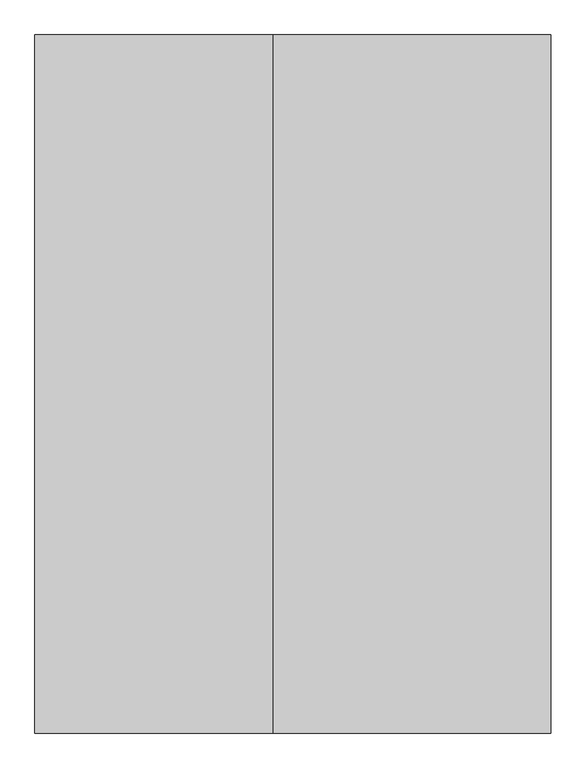
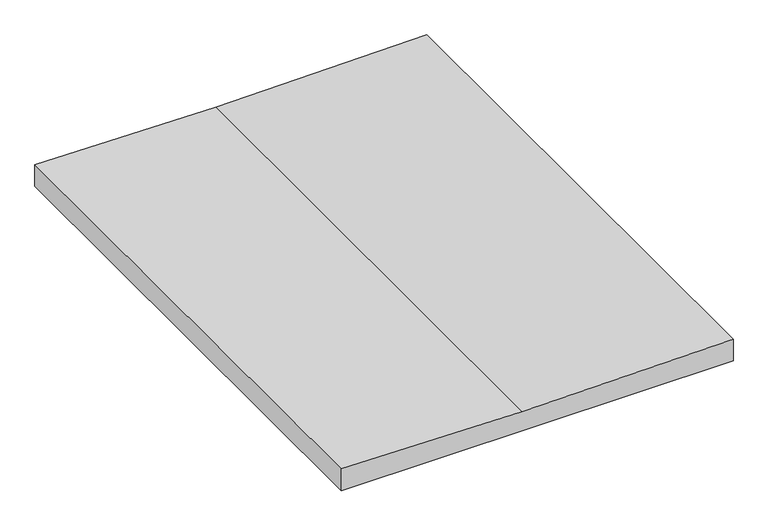
"""IFC4 building model written with IfcOpenShell, lengths in millimetres: proxy geometry, FIRESTONE INSULATION001 1:FIRESTONE INSULATION001 15434:299739 : FIRESTONE INSULATION001 1:FIRESTONE INSULATION001 15434:299739."""

from ifc_helpers import new_model, si_unit, frame, origin, place, context, project, spatial, polyline, outline, extrude, source, transform, mapped, element, save


def generic_models_139e72a4(model_context):
    return source(origin(), model_context, "Body", "SweptSolid", [
        extrude(outline(polyline([(40218.4000089, 2209.6354065), (40131.746, 2209.6354065), (40131.746, 3686.9275669), (40218.4000089, 3686.9275669), (40208.6021556, 2890.4461596), (40218.4000089, 2209.6354065)])), frame((0.0, -774.3081162, 0.0), z_axis=(0.0, 1.0, 0.0), x_axis=(0.0, 0.0, 1.0)), (0.0, 0.0, 1.0), 2000.0),
    ])


if __name__ == "__main__":
    model = new_model("IFC4")
    model_context = context("Model", 3, world=origin())
    ifc_project = project(units=[si_unit("LENGTHUNIT", "METRE", prefix="MILLI")], contexts=[model_context])
    site = spatial("IfcSite", under=ifc_project)
    building = spatial("IfcBuilding", under=site)
    placement = place(None, origin())
    generic_models_shape = generic_models_139e72a4(model_context)
    element("IfcBuildingElementProxy", 1, Name="FIRESTONE INSULATION001 1:FIRESTONE INSULATION001 15434:299739 : FIRESTONE INSULATION001 1:FIRESTONE INSULATION001 15434:299739", ObjectType="FIRESTONE INSULATION001 1:FIRESTONE INSULATION001 15434:299739 : FIRESTONE INSULATION001 1:FIRESTONE INSULATION001 15434:299739", at=placement, inside=building, context=model_context, shape_type="MappedRepresentation", body=[
        mapped(generic_models_shape, transform((0.0, 0.0, 0.0), x_axis=(1.0, 0.0, 0.0), y_axis=(0.0, 1.0, 0.0), z_axis=(0.0, 0.0, 1.0))),
    ])
    save(model, "model.ifc")

# Revit data of these elements
# Type "FIRESTONE INSULATION001 1:FIRESTONE INSULATION001 15434:299739 : FIRESTONE INSULATION001 1:FIRESTONE INSULATION001 15434:299739"
#   NameOverride = "FIRESTONE INSULATION001 1:FIRESTONE INSULATION001 15434:299739"
#   ObjectTypeOverride = "FIRESTONE INSULATION001 1:FIRESTONE INSULATION001 15434"
#   Reference = "FIRESTONE INSULATION001 15434"
#   Category = "Generic Models"
#   Tag = "299739"
# Element 1 (IfcBuildingElementProxy, "FIRESTONE INSULATION001 1:FIRESTONE INSULATION001 15434:299739 : FIRESTONE INSULATION001 1:FIRESTONE INSULATION001 15434:299739")
#   Materials on its faces: "TAPERED 2X SLEEPERS - SLOPED TO DRAIN"
# Materials
#   "TAPERED 2X SLEEPERS - SLOPED TO DRAIN": class "Unassigned", colour RGB 234 198 178, transparency 0
